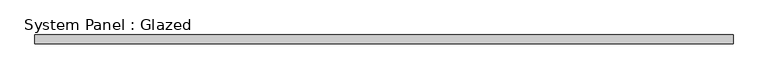
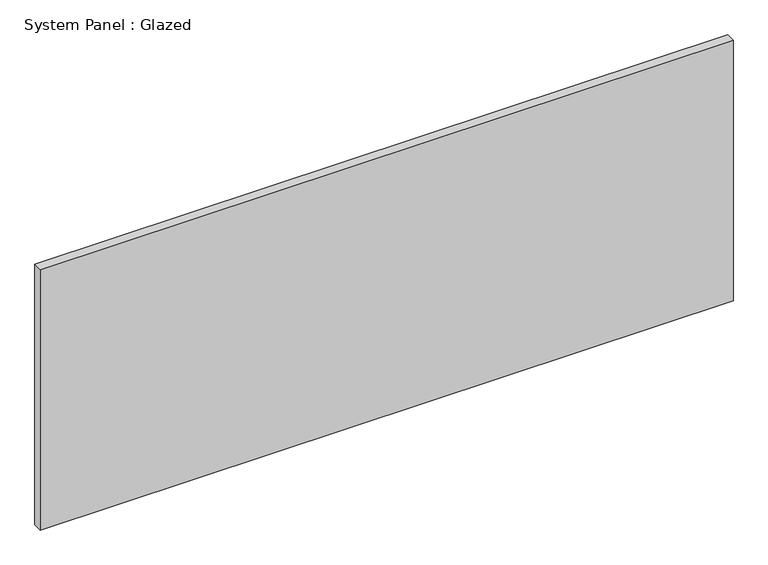
"""IFC4 building model written with IfcOpenShell, lengths in millimetres: plate geometry, System Panel : Glazed."""

from ifc_helpers import new_model, si_unit, origin, origin_with_axes, place, context, project, spatial, polyline, outline, extrude, source, transform, mapped, element, save


def system_panel_glazed_d82c9dbb(model_context):
    return source(origin(), model_context, "Body", "SweptSolid", [
        extrude(outline(polyline([(975.0000002, 24.5), (-975.0000002, 24.5), (-975.0000002, 49.5), (975.0000002, 49.5), (975.0000002, 24.5)])), origin_with_axes(), (0.0, 0.0, 1.0), 775.0),
    ])


if __name__ == "__main__":
    model = new_model("IFC4")
    model_context = context("Model", 3, world=origin())
    ifc_project = project(units=[si_unit("LENGTHUNIT", "METRE", prefix="MILLI")], contexts=[model_context])
    site = spatial("IfcSite", under=ifc_project)
    building = spatial("IfcBuilding", under=site)
    placement = place(None, origin())
    system_panel_glazed_shape = system_panel_glazed_d82c9dbb(model_context)
    element("IfcPlate", 1, ObjectType="System Panel : Glazed", at=placement, inside=building, context=model_context, shape_type="MappedRepresentation", body=[
        mapped(system_panel_glazed_shape, transform((0.0, 0.0, 0.0), x_axis=(1.0, 0.0, 0.0), y_axis=(0.0, 1.0, 0.0), z_axis=(0.0, 0.0, 1.0))),
    ])
    save(model, "model.ifc")

# Revit data of these elements
# Element 1 (IfcPlate, "System Panel : Glazed")
#   Materials on its faces: "Glass"
# Materials
#   "Glass": class "Glass", colour RGB 0 128 192, transparency 0.9
